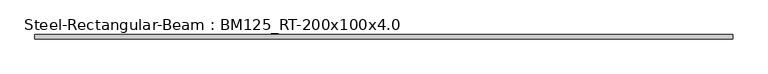
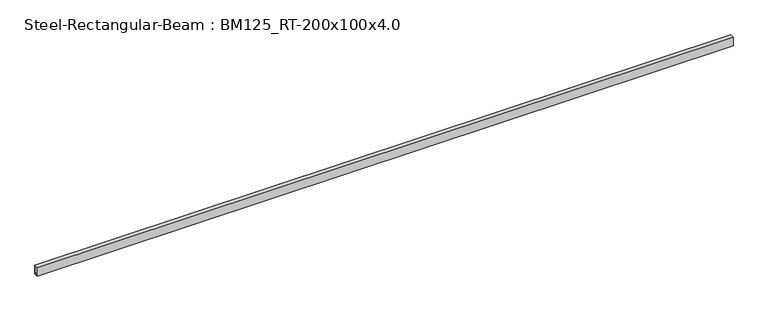
"""IFC4 building model written with IfcOpenShell, lengths in millimetres: beam geometry, Steel-Rectangular-Beam : BM125_RT-200x100x4.0."""

import ifcopenshell
import ifcopenshell.guid

model = None  # the IFC model being written
_history = None  # IfcOwnerHistory: only IFC2X3 demands one
_inside = {}  # id of a spatial element -> (the spatial element, [elements in it])
_under = {}  # id of a project, library or spatial element -> (it, [spatial elements below it])
_declared = {}  # id of a project -> (the project, [libraries it declares])
_typed = {}  # id of a type object -> (the type object, [elements of that type])
_made_of = {}  # id of a material, layer set ... -> (it, [elements and type objects made of it])


def new_model(schema):
    """Start an empty IFC model of exactly this schema.

    Asked for "IFC4X3", IfcOpenShell would pick the latest addendum, in which some entities
    have other attributes; the version numbers below select the first issue.
    IFC2X3 requires an IfcOwnerHistory on every rooted entity: one is made here for all.
    """
    global model, _history
    if schema == "IFC4X3":
        model = ifcopenshell.file(schema_version=(4, 3, 0, 0))
    else:
        model = ifcopenshell.file(schema=schema)
    _inside.clear()
    _under.clear()
    _declared.clear()
    _typed.clear()
    _made_of.clear()
    _history = None
    if model.schema == "IFC2X3":
        org = make("IfcOrganization", Name="unknown")
        user = make(
            "IfcPersonAndOrganization",
            ThePerson=make("IfcPerson", FamilyName="unknown"),
            TheOrganization=org,
        )
        app = make(
            "IfcApplication",
            ApplicationDeveloper=org,
            Version="unknown",
            ApplicationFullName="unknown",
            ApplicationIdentifier="unknown",
        )
        _history = make(
            "IfcOwnerHistory",
            OwningUser=user,
            OwningApplication=app,
            ChangeAction="ADDED",
            CreationDate=0,
        )
    return model


def make(cls, **values):
    """One entity of the class cls with the attributes given. An attribute that is None is left unset."""
    return model.create_entity(
        cls, **{name: value for name, value in values.items() if value is not None}
    )


def rooted(cls, **values):
    """An entity with a GlobalId (a new one), such as an element, a storey or a relation."""
    return make(cls, GlobalId=ifcopenshell.guid.new(), OwnerHistory=_history, **values)


def si_unit(unit_type, name, prefix=None):
    """IfcSIUnit, for example si_unit("LENGTHUNIT", "METRE", prefix="MILLI")."""
    return make("IfcSIUnit", UnitType=unit_type, Prefix=prefix, Name=name)


def assignment(units):
    """IfcUnitAssignment: the units of a project."""
    return None if units is None else make("IfcUnitAssignment", Units=units)


def point(xyz):
    """IfcCartesianPoint."""
    return None if xyz is None else make("IfcCartesianPoint", Coordinates=xyz)


def direction(xyz):
    """IfcDirection."""
    return None if xyz is None else make("IfcDirection", DirectionRatios=xyz)


def frame(location, z_axis=None, x_axis=None):
    """IfcAxis2Placement3D, a coordinate frame: its origin and axes. An axis left out is left unset."""
    return make(
        "IfcAxis2Placement3D",
        Location=point(location),
        Axis=direction(z_axis),
        RefDirection=direction(x_axis),
    )


def origin():
    """The frame at (0, 0, 0) with its axes left unset."""
    return frame((0.0, 0.0, 0.0))


def place(relative_to, where):
    """IfcLocalPlacement: puts the frame where relative to a parent placement (None: the world)."""
    return make(
        "IfcLocalPlacement", PlacementRelTo=relative_to, RelativePlacement=where
    )


def context(
    kind, dimensions, precision=None, world=None, true_north=None, identifier=None
):
    """IfcGeometricRepresentationContext, for example the 3D "Model" context."""
    return make(
        "IfcGeometricRepresentationContext",
        ContextIdentifier=identifier,
        ContextType=kind,
        CoordinateSpaceDimension=dimensions,
        Precision=precision,
        WorldCoordinateSystem=world,
        TrueNorth=true_north,
    )


def project(units=None, contexts=None):
    """IfcProject with its units and contexts."""
    return rooted(
        "IfcProject",
        Name="project",
        RepresentationContexts=contexts,
        UnitsInContext=assignment(units),
    )


def spatial(cls, under=None, at=None, **own):
    """A site, building, storey or space (cls), placed at a placement, below another one or the project."""
    s = rooted(cls, ObjectPlacement=at, **own)
    if under is not None:
        _under.setdefault(under.id(), (under, []))[1].append(s)
    return s


def polyline(points):
    """IfcPolyline through the points."""
    return make("IfcPolyline", Points=[point(p) for p in points])


def outline(outer, holes=None, kind="AREA"):
    """IfcArbitraryClosedProfileDef: a profile drawn as a closed curve; with holes, ...WithVoids."""
    if holes is None:
        return make("IfcArbitraryClosedProfileDef", ProfileType=kind, OuterCurve=outer)
    return make(
        "IfcArbitraryProfileDefWithVoids",
        ProfileType=kind,
        OuterCurve=outer,
        InnerCurves=holes,
    )


def extrude(swept, where, along, depth):
    """IfcExtrudedAreaSolid: the profile swept, set in the frame where, extruded along a direction by depth."""
    return make(
        "IfcExtrudedAreaSolid",
        SweptArea=swept,
        Position=where,
        ExtrudedDirection=direction(along),
        Depth=depth,
    )


def shape(context_of_items, identifier, shape_type, items):
    """IfcShapeRepresentation: the items that make up one representation, for example the "Body"."""
    return make(
        "IfcShapeRepresentation",
        ContextOfItems=context_of_items,
        RepresentationIdentifier=identifier,
        RepresentationType=shape_type,
        Items=items,
    )


def source(mapping_origin, context_of_items, identifier, shape_type, items):
    """IfcRepresentationMap: a shape defined once, which mapped items show again and again."""
    return make(
        "IfcRepresentationMap",
        MappingOrigin=mapping_origin,
        MappedRepresentation=shape(context_of_items, identifier, shape_type, items),
    )


def transform(
    local_origin,
    x_axis=None,
    y_axis=None,
    z_axis=None,
    scale=None,
    scale2=None,
    scale3=None,
    uniform=True,
):
    """IfcCartesianTransformationOperator3D, or its non-uniform kind. x_axis, y_axis, z_axis: its Axis1, 2, 3."""
    if uniform:
        return make(
            "IfcCartesianTransformationOperator3D",
            Axis1=direction(x_axis),
            Axis2=direction(y_axis),
            LocalOrigin=point(local_origin),
            Scale=scale,
            Axis3=direction(z_axis),
        )
    return make(
        "IfcCartesianTransformationOperator3DnonUniform",
        Axis1=direction(x_axis),
        Axis2=direction(y_axis),
        LocalOrigin=point(local_origin),
        Scale=scale,
        Axis3=direction(z_axis),
        Scale2=scale2,
        Scale3=scale3,
    )


def mapped(mapping_source, mapping_target):
    """IfcMappedItem: shows the shape of a source again, moved by a transform."""
    return make(
        "IfcMappedItem", MappingSource=mapping_source, MappingTarget=mapping_target
    )


def made_of(thing, what):
    """Note that an element or type object is made of a material, layer set ...; save() writes the relation."""
    if what is not None:
        _made_of.setdefault(what.id(), (what, []))[1].append(thing)
    return thing


def element(
    cls,
    number,
    at=None,
    inside=None,
    cuts=None,
    type_object=None,
    material=None,
    context=None,
    identifier="Body",
    shape_type=None,
    held_by="IfcProductDefinitionShape",
    body=None,
    shapes=None,
    **own,
):
    """One element of the class cls, such as IfcWall. Its Tag is "e" and its number.

    at: its placement. inside: the storey or other place that contains it. cuts: it is an
    opening in that element (IfcRelVoidsElement). A single representation is given by context,
    identifier, shape_type and body (its items); several are given by shapes. held_by: the class
    of the entity that holds the representations. save() writes the other relations.
    """
    e = rooted(cls, Tag="e%d" % number, ObjectPlacement=at, **own)
    if body is not None:
        shapes = [shape(context, identifier, shape_type, body)]
    if shapes is not None:
        e.Representation = make(held_by, Representations=shapes)
    if inside is not None:
        _inside.setdefault(inside.id(), (inside, []))[1].append(e)
    if cuts is not None:
        rooted(
            "IfcRelVoidsElement", RelatingBuildingElement=cuts, RelatedOpeningElement=e
        )
    if type_object is not None:
        _typed.setdefault(type_object.id(), (type_object, []))[1].append(e)
    return made_of(e, material)


def aggregate(whole, parts):
    """IfcRelAggregates: a whole, such as a stair, and the parts it consists of."""
    return rooted("IfcRelAggregates", RelatingObject=whole, RelatedObjects=parts)


def save(model, path):
    """Write the relations noted so far, then the file.

    IfcRelAggregates (storeys below a building ...), IfcRelContainedInSpatialStructure (elements
    in a storey), IfcRelDefinesByType, IfcRelAssociatesMaterial and IfcRelDeclares: one each for
    every whole, place, type object, material and project.
    """
    for whole, parts in _under.values():
        aggregate(whole, parts)
    for where, things in _inside.values():
        rooted(
            "IfcRelContainedInSpatialStructure",
            RelatedElements=things,
            RelatingStructure=where,
        )
    for kind, things in _typed.values():
        rooted("IfcRelDefinesByType", RelatedObjects=things, RelatingType=kind)
    for what, things in _made_of.values():
        rooted("IfcRelAssociatesMaterial", RelatedObjects=things, RelatingMaterial=what)
    for by, libraries in _declared.values():
        rooted("IfcRelDeclares", RelatingContext=by, RelatedDefinitions=libraries)
    model.write(path)


def steel_rectangular_beam_bm125_rt_200x100x4_0_52f716dd(model_context):
    return source(origin(), model_context, "Body", "SweptSolid", [
        extrude(outline(polyline([(-50.0, 100.0), (50.0, 100.0), (50.0, -100.0), (-50.0, -100.0), (-50.0, 100.0)]), holes=[polyline([(46.0, -96.0), (46.0, 96.0), (-46.0, 96.0), (-46.0, -96.0), (46.0, -96.0)])]), frame((-8000.0, 0.0, 0.0), z_axis=(1.0, 0.0, 0.0), x_axis=(0.0, 1.0, 0.0)), (0.0, 0.0, 1.0), 16000.0),
        extrude(outline(polyline([(-50.0, 100.0), (50.0, 100.0), (50.0, -100.0), (-50.0, -100.0), (-50.0, 100.0)]), holes=[polyline([(46.0, -96.0), (46.0, 96.0), (-46.0, 96.0), (-46.0, -96.0), (46.0, -96.0)])]), frame((-8000.0, 0.0, 0.0), z_axis=(1.0, 0.0, 0.0), x_axis=(0.0, 1.0, 0.0)), (0.0, 0.0, 1.0), 16000.0),
        extrude(outline(polyline([(-50.0, 100.0), (50.0, 100.0), (50.0, -100.0), (-50.0, -100.0), (-50.0, 100.0)]), holes=[polyline([(46.0, -96.0), (46.0, 96.0), (-46.0, 96.0), (-46.0, -96.0), (46.0, -96.0)])]), frame((-8000.0, 0.0, 0.0), z_axis=(1.0, 0.0, 0.0), x_axis=(0.0, 1.0, 0.0)), (0.0, 0.0, 1.0), 16000.0),
        extrude(outline(polyline([(-50.0, 100.0), (50.0, 100.0), (50.0, -100.0), (-50.0, -100.0), (-50.0, 100.0)]), holes=[polyline([(46.0, -96.0), (46.0, 96.0), (-46.0, 96.0), (-46.0, -96.0), (46.0, -96.0)])]), frame((-8000.0, 0.0, 0.0), z_axis=(1.0, 0.0, 0.0), x_axis=(0.0, 1.0, 0.0)), (0.0, 0.0, 1.0), 16000.0),
    ])


if __name__ == "__main__":
    model = new_model("IFC4")
    model_context = context("Model", 3, world=origin())
    ifc_project = project(units=[si_unit("LENGTHUNIT", "METRE", prefix="MILLI")], contexts=[model_context])
    site = spatial("IfcSite", under=ifc_project)
    building = spatial("IfcBuilding", under=site)
    placement = place(None, origin())
    steel_rectangular_beam_bm125_rt_200x100x4_0_shape = steel_rectangular_beam_bm125_rt_200x100x4_0_52f716dd(model_context)
    element("IfcBeam", 1, ObjectType="Steel-Rectangular-Beam : BM125_RT-200x100x4.0", at=placement, inside=building, context=model_context, shape_type="MappedRepresentation", body=[
        mapped(steel_rectangular_beam_bm125_rt_200x100x4_0_shape, transform((0.0, 0.0, 0.0), x_axis=(1.0, 0.0, 0.0), y_axis=(0.0, 1.0, 0.0), z_axis=(0.0, 0.0, 1.0))),
    ])
    save(model, "model.ifc")

# Revit data of these elements
# Type "Steel-Rectangular-Beam : BM125_RT-200x100x4.0"
#   t = 4 mm
#   Mass per Unit Length = 18.35 kg/m
#   Surface Area = 0.60 m²/m
#   Sectional Area = 1856.0 cm²
#   Length [instance default] = 3000 mm
#   H = 200 mm
#   B = 100 mm
#   hec_material4 [instance default] = none
#   hec_material3 [instance default] = none
#   hec_material2 [instance default] = none
#   hec_material1 [instance default] = none
#   Structural Material [instance default] = none
# Element 1 (IfcBeam, "Steel-Rectangular-Beam : BM125_RT-200x100x4.0")
#   hec_material2 = S01AA010-00001_Main Steel Structure Fabrication Work_Shelter/Building_Steel Painting/Coating_for Non-Fireproofed Steel Surface, Surface Preparation, Primer, Second & Final Coat
#   hec_material1 = S03AA007-00001_Main Steel Structure Erection Work_Girth & Purlin
#   Structural Material = S01AA007-00001_Main Steel Structure Fabrication Work_Shelter/Building_Girth & Purlin
#   Materials on its faces: "S01AA010-00001_Main Steel Structure Fabrication Work_Shelter/Building_Steel Painting/Coating_for Non-Fireproofed Steel Surface, Surface Preparation, Primer, Second & Final Coat"
# Materials
#   "S01AA010-00001_Main Steel Structure Fabrication Work_Shelter/Building_Steel Painting/Coating_for Non-Fireproofed Steel Surface, Surface Preparation, Primer, Second & Final Coat": class "Metal", colour RGB 120 120 120, transparency 0, Description = "Paint finished steel", W00) Work Master Code = "S01AA010-00001", W01) Work Master_Lv1 = "Main Steel Structure Fabrication Work", W02) Work Master_Lv2 = "Shelter/Building", W03) Work Master_Spec.1 = "Steel Painting/Coating", W04) Work Master_Spec.2 = "for Non-Fireproofed Steel Surface, Surface Preparation, Primer, Second & Final Coat", Cost = 0
#   "S03AA007-00001_Main Steel Structure Erection Work_Girth & Purlin": class "Metal", colour RGB 120 120 120, transparency 0, Comments = "(30KG/M>Weight)", Description = "Structural steel 50ksi", W00) Work Master Code = "S03AA007-00001", W01) Work Master_Lv1 = "Main Steel Structure Erection Work", W02) Work Master_Lv2 = "Shelter/Building", W03) Work Master_Spec.1 = "Girth & Purlin", Cost = 0
#   "S01AA007-00001_Main Steel Structure Fabrication Work_Shelter/Building_Girth & Purlin": class "Metal", colour RGB 120 120 120, transparency 0, Comments = "(30KG/M>Weight)", Description = "Structural steel 50ksi", W00) Work Master Code = "S01AA007-00001", W01) Work Master_Lv1 = "Main Steel Structure Fabrication Work", W02) Work Master_Lv2 = "Shelter/Building", W03) Work Master_Spec.1 = "Girth & Purlin", Cost = 0
